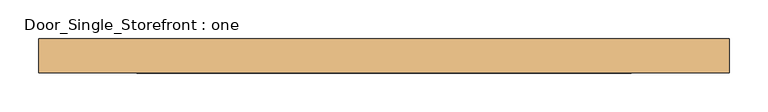
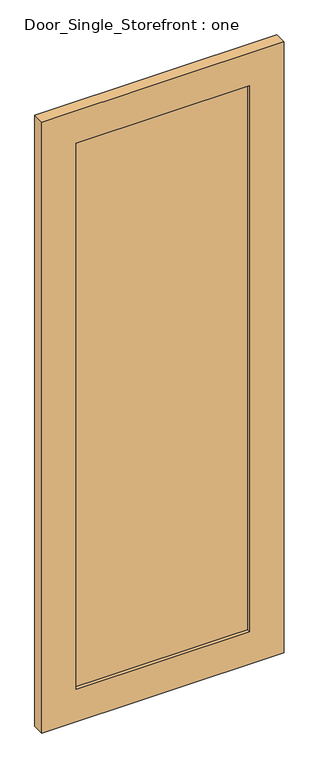
"""IFC4 building model written with IfcOpenShell, lengths in millimetres: door geometry, Door_Single_Storefront : one."""

from ifc_helpers import new_model, si_unit, frame, origin, place, context, project, spatial, polyline, outline, extrude, source, transform, mapped, element, save


def door_single_storefront_one_50d196f4(model_context):
    return source(origin(), model_context, "Body", "SweptSolid", [
        extrude(outline(polyline([(319.88125, -6.35), (-319.88125, -6.35), (-319.88125, 12.7), (319.88125, 12.7), (319.88125, -6.35)])), frame((0.0, 0.0, 127.0), z_axis=(0.0, 0.0, 1.0), x_axis=(1.0, 0.0, 0.0)), (0.0, 0.0, 1.0), 2127.25),
        extrude(outline(polyline([(2381.25, -446.88125), (0.0, -446.88125), (0.0, 446.88125), (2381.25, 446.88125), (2381.25, -446.88125)]), holes=[polyline([(127.0, 319.88125), (127.0, -319.88125), (2254.25, -319.88125), (2254.25, 319.88125), (127.0, 319.88125)])]), frame((0.0, -19.05, 0.0), z_axis=(0.0, 1.0, 0.0), x_axis=(0.0, 0.0, 1.0)), (0.0, 0.0, 1.0), 44.45),
    ])


if __name__ == "__main__":
    model = new_model("IFC4")
    model_context = context("Model", 3, world=origin())
    ifc_project = project(units=[si_unit("LENGTHUNIT", "METRE", prefix="MILLI")], contexts=[model_context])
    site = spatial("IfcSite", under=ifc_project)
    building = spatial("IfcBuilding", under=site)
    placement = place(None, origin())
    door_single_storefront_one_shape = door_single_storefront_one_50d196f4(model_context)
    element("IfcDoor", 1, ObjectType="Door_Single_Storefront : one", at=placement, inside=building, context=model_context, shape_type="MappedRepresentation", body=[
        mapped(door_single_storefront_one_shape, transform((0.0, 0.0, 0.0), x_axis=(1.0, 0.0, 0.0), y_axis=(0.0, 1.0, 0.0), z_axis=(0.0, 0.0, 1.0))),
    ])
    save(model, "model.ifc")

# Revit data of these elements
# Type "Door_Single_Storefront : one"
#   Type Mark = "27"
#   Analytic Construction = "<None>"
#   Stile_Width = 0' - 5"
#   Door_Thickness = 0' - 1 3/4"
#   Door_Offset = 0' - 1"
#   Glass_Material = SAFETY GLAZING
#   Frame_Material = INTERIOR GRADE ALUMINUM STOREFRONT W/ SAFETY GLAZING
#   Function = (empty or 0)
# Element 1 (IfcDoor, "Door_Single_Storefront : one")
#   Materials on its faces: "INTERIOR GRADE ALUMINUM STOREFRONT W/ SAFETY GLAZING", "SAFETY GLAZING"
# Materials
#   "SAFETY GLAZING": class "Glass", colour RGB 142 168 196, transparency 0.75, Description = "Soda Lime Glass", Cost = 0
#   "INTERIOR GRADE ALUMINUM STOREFRONT W/ SAFETY GLAZING": class "Metal", colour RGB 226 226 226, transparency 0, Description = "Aluminum 6061", Cost = 0
